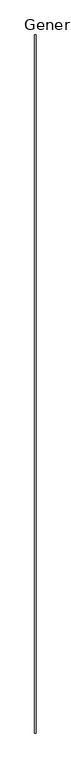
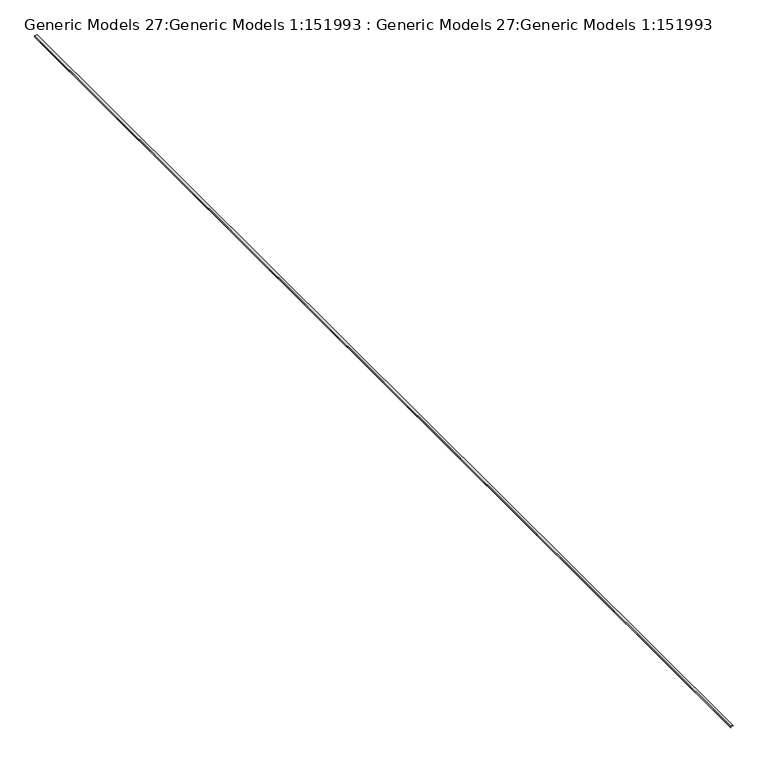
"""IFC4 building model written with IfcOpenShell, lengths in millimetres: proxy geometry, Generic Models 27:Generic Models 1:151993 : Generic Models 27:Generic Models 1:151993."""

from ifc_helpers import new_model, si_unit, frame, origin, place, context, project, spatial, polyline, outline, extrude, source, transform, mapped, element, save


def generic_models_27_generic_models_1_151993_generic_models_27_01759fe1(model_context):
    return source(origin(), model_context, "Body", "SweptSolid", [
        extrude(outline(polyline([(3067.05, 8352.826963), (3044.825, 8352.826963), (3044.825, 8357.576763), (3047.8274564, 8357.576763), (3047.8274564, 8356.306763), (3046.095, 8356.306763), (3046.095, 8354.096963), (3065.78, 8354.096963), (3065.78, 8390.926963), (3067.05, 8390.926963), (3067.05, 8352.826963)])), frame((0.0, -2153.5974793, 0.0), z_axis=(0.0, 1.0, 0.0), x_axis=(0.0, 0.0, 1.0)), (0.0, 0.0, 1.0), 19050.0),
    ])


if __name__ == "__main__":
    model = new_model("IFC4")
    model_context = context("Model", 3, world=origin())
    ifc_project = project(units=[si_unit("LENGTHUNIT", "METRE", prefix="MILLI")], contexts=[model_context])
    site = spatial("IfcSite", under=ifc_project)
    building = spatial("IfcBuilding", under=site)
    placement = place(None, origin())
    generic_models_27_generic_models_1_151993_generic_models_27_shape = generic_models_27_generic_models_1_151993_generic_models_27_01759fe1(model_context)
    element("IfcBuildingElementProxy", 1, Name="Generic Models 27:Generic Models 1:151993 : Generic Models 27:Generic Models 1:151993", ObjectType="Generic Models 27:Generic Models 1:151993 : Generic Models 27:Generic Models 1:151993", at=placement, inside=building, context=model_context, shape_type="MappedRepresentation", body=[
        mapped(generic_models_27_generic_models_1_151993_generic_models_27_shape, transform((0.0, 0.0, 0.0), x_axis=(1.0, 0.0, 0.0), y_axis=(0.0, 1.0, 0.0), z_axis=(0.0, 0.0, 1.0))),
    ])
    save(model, "model.ifc")

# Revit data of these elements
# Type "Generic Models 27:Generic Models 1:151993 : Generic Models 27:Generic Models 1:151993"
#   NameOverride = "Generic Models 27:Generic Models 1:151993"
#   ObjectTypeOverride = "Generic Models 27:Generic Models 1"
#   Reference = "Generic Models 1"
#   Category = "Generic Models"
#   Tag = "151993"
# Element 1 (IfcBuildingElementProxy, "Generic Models 27:Generic Models 1:151993 : Generic Models 27:Generic Models 1:151993")
#   Materials on its faces: "_CONTINUOUS 16 GA. COPPER  J BEAD 1960"
# Materials
#   "_CONTINUOUS 16 GA. COPPER  J BEAD 1960": class "Unassigned", colour RGB 253 192 103, transparency 0
